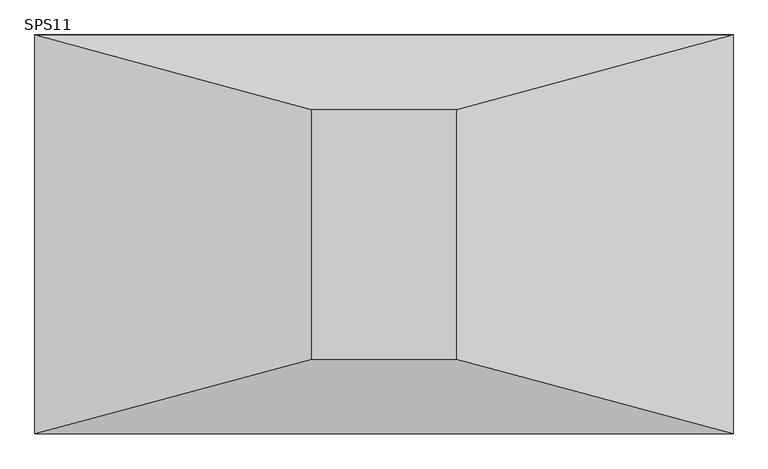
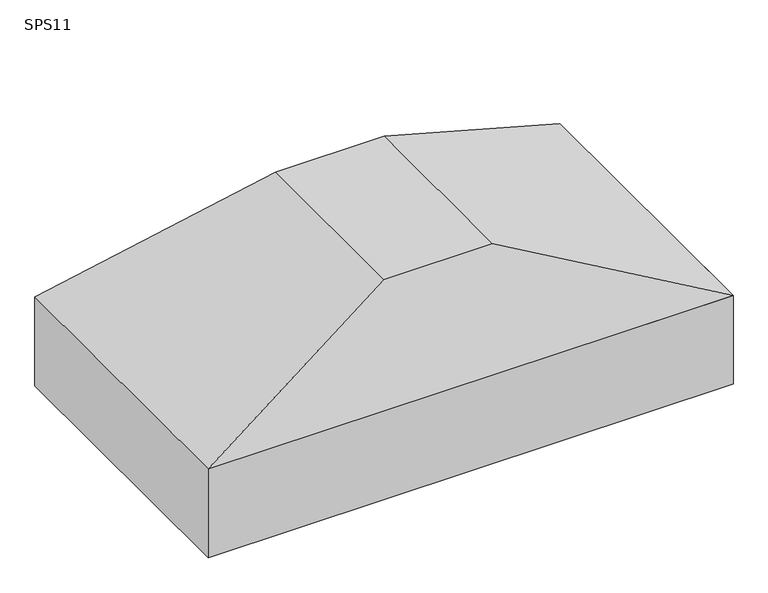
"""IFC4 building model written with IfcOpenShell, lengths in millimetres: fastener geometry, TQS - Sapata : SPS11."""

from ifc_helpers import new_model, si_unit, frame, origin, place, context, project, spatial, polyline, outline, extrude, faceted_brep, source, transform, mapped, element, save


def sps11_3ae28187(model_context):
    return source(origin(), model_context, "Body", "SolidModel", [
        faceted_brep([(-55.0, 50.0, 0.0), (-345.0, 50.0, 0.0), (-345.0, -450.0, 0.0), (-55.0, -450.0, 0.0), (500.0, 200.0, -250.0), (500.0, -600.0, -250.0), (-900.0, -600.0, -250.0), (-900.0, 200.0, -250.0)], [[[0, 1, 2, 3]], [[4, 5, 6, 7]], [[4, 7, 1, 0]], [[7, 6, 2, 1]], [[6, 5, 3, 2]], [[5, 4, 0, 3]]]),
        extrude(outline(polyline([(500.0, 200.0), (500.0, -600.0), (-900.0, -600.0), (-900.0, 200.0), (500.0, 200.0)])), frame((0.0, 0.0, -500.0), z_axis=(0.0, 0.0, 1.0), x_axis=(1.0, 0.0, 0.0)), (0.0, 0.0, 1.0), 250.0),
    ])


if __name__ == "__main__":
    model = new_model("IFC4")
    model_context = context("Model", 3, world=origin())
    ifc_project = project(units=[si_unit("LENGTHUNIT", "METRE", prefix="MILLI")], contexts=[model_context])
    site = spatial("IfcSite", under=ifc_project)
    building = spatial("IfcBuilding", under=site)
    placement = place(None, origin())
    sps11_shape = sps11_3ae28187(model_context)
    element("IfcFastener", 1, ObjectType="TQS - Sapata : SPS11", at=placement, inside=building, context=model_context, shape_type="MappedRepresentation", body=[
        mapped(sps11_shape, transform((0.0, 0.0, 0.0), x_axis=(1.0, 0.0, 0.0), y_axis=(0.0, 1.0, 0.0), z_axis=(0.0, 0.0, 1.0))),
    ])
    save(model, "model.ifc")

# Revit data of these elements
# Type "TQS - Sapata : SPS11"
#   TY = 0.50 m
#   TX = 0.29 m
#   HS = 0.50 m
#   H0 = 0.25 m
#   EXCYABS = 0.40 m
#   EXCY = 0.00 m
#   EXCXABS = 0.70 m
#   EXCX = 0.00 m
#   DIMY = 0.80 m
#   DIMX = 1.40 m
#   Material estrutural = Concreto - Concreto concretado no local
#   Width = 0
#   Length = 0
# Element 1 (IfcFastener, "TQS - Sapata : SPS11")
#   Materials on its faces: "Concreto - Concreto concretado no local"
# Materials
#   "Concreto - Concreto concretado no local": class "Concreto", colour RGB 192 192 192, transparency 0
